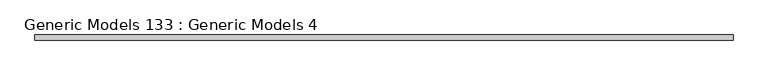
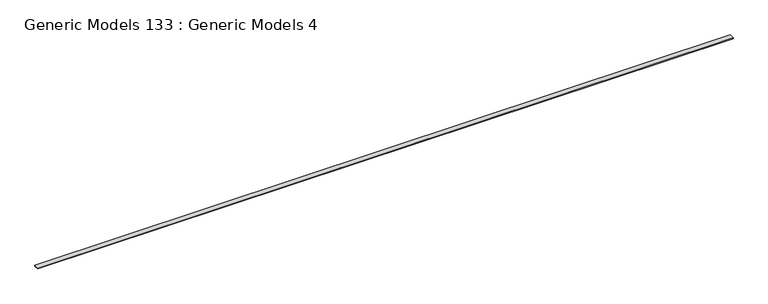
"""IFC4 building model written with IfcOpenShell, lengths in millimetres: proxy geometry, Generic Models 133 : Generic Models 4."""

from ifc_helpers import new_model, si_unit, frame, origin, place, context, project, spatial, polyline, outline, extrude, source, transform, mapped, element, save


def generic_models_133_generic_models_4_29c974bb(model_context):
    return source(origin(), model_context, "Body", "SweptSolid", [
        extrude(outline(polyline([(21700.7658099, 12408.398069), (21700.7658099, 12305.9629664), (7781.5658099, 12305.9629664), (7781.5658099, 12408.398069), (21700.7658099, 12408.398069)])), frame((0.0, 0.0, 129277.2366834), z_axis=(0.0, 0.0, 1.0), x_axis=(1.0, 0.0, 0.0)), (0.0, 0.0, 1.0), 18.3199747),
    ])


if __name__ == "__main__":
    model = new_model("IFC4")
    model_context = context("Model", 3, world=origin())
    ifc_project = project(units=[si_unit("LENGTHUNIT", "METRE", prefix="MILLI")], contexts=[model_context])
    site = spatial("IfcSite", under=ifc_project)
    building = spatial("IfcBuilding", under=site)
    placement = place(None, origin())
    generic_models_133_generic_models_4_shape = generic_models_133_generic_models_4_29c974bb(model_context)
    element("IfcBuildingElementProxy", 1, Name="Generic Models 133 : Generic Models 4", ObjectType="Generic Models 133 : Generic Models 4", at=placement, inside=building, context=model_context, shape_type="MappedRepresentation", body=[
        mapped(generic_models_133_generic_models_4_shape, transform((0.0, 0.0, 0.0), x_axis=(1.0, 0.0, 0.0), y_axis=(0.0, 1.0, 0.0), z_axis=(0.0, 0.0, 1.0))),
    ])
    save(model, "model.ifc")

# Revit data of these elements
# Element 1 (IfcBuildingElementProxy, "Generic Models 133 : Generic Models 4")
#   Materials on its faces: "_2X BLOCKING AS REQUIRED"
# Materials
#   "_2X BLOCKING AS REQUIRED": class "Generic", colour RGB 177 130 114, transparency 0, Cost = 0
